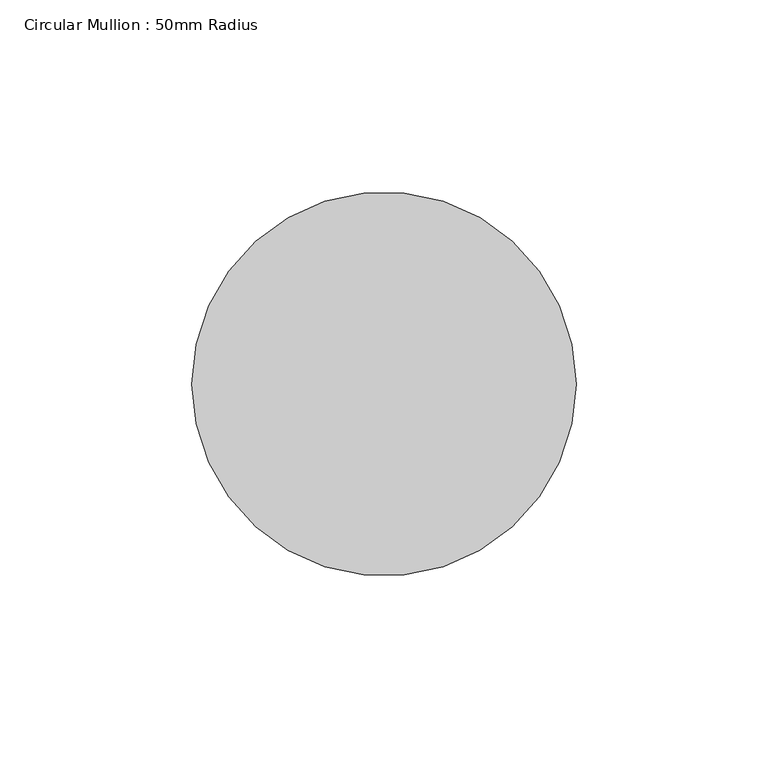
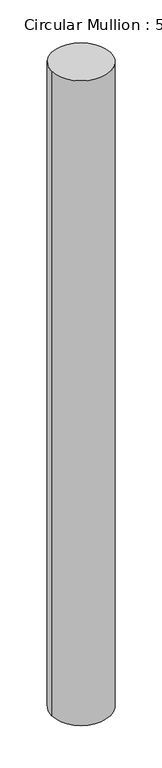
"""IFC4 building model written with IfcOpenShell, lengths in millimetres: member geometry, Circular Mullion : 50mm Radius."""

from ifc_helpers import new_model, si_unit, frame, origin, place, context, project, spatial, ellipse_curve, source, transform, mapped, element, save
from ifc_brep_helpers import plane_surface, cylinder_surface, advanced_brep


def circular_mullion_50mm_radius_0a69bc8c(model_context):
    return source(origin(), model_context, "Body", "AdvancedBrep", [
        advanced_brep(
        [(-100.0, 0.0, 0.8319874), (0.0, 0.0, 0.0), (0.0, 0.0, -1158.0703497), (-100.0, 0.0, -1158.8687099)],
        [
            (0, 1, ellipse_curve(frame((-50.0, 0.0, 0.4159937), z_axis=(-0.008318788476697321, -0.013847806669910945, -0.9998695094904698), x_axis=(-0.5148884069821343, -0.8571049902807197, 0.01615437994128195)), 50.0065254, 50.0)),
            (1, 2),
            (2, 3, ellipse_curve(frame((-50.0, 0.0, -1158.4695298), z_axis=(-0.007982642623571047, -0.013288244084562615, 0.9998798427740674), x_axis=(0.5148937281644346, 0.857113848145521, 0.015501613274298874)), 50.0060086, 50.0)),
            (3, 0),
            (1, 0, ellipse_curve(frame((-50.0, 0.0, 0.4159937), z_axis=(-0.008318788476697321, -0.013847806669910945, -0.9998695094904698), x_axis=(-0.5148884069821343, -0.8571049902807197, 0.01615437994128195)), 50.0065254, 50.0)),
            (3, 2, ellipse_curve(frame((-50.0, 0.0, -1158.4695298), z_axis=(-0.007982642623571047, -0.013288244084562615, 0.9998798427740674), x_axis=(0.5148937281644346, 0.857113848145521, 0.015501613274298874)), 50.0060086, 50.0)),
        ],
        [
            cylinder_surface(frame((-50.0, 0.0, 0.0), z_axis=(0.0, 0.0, 1.0), x_axis=(1.0, 0.0, 0.0)), 50.0),
            plane_surface(frame((-261.2796956, 156.958468, 0.0), z_axis=(0.008318788476697321, 0.013847806669910945, 0.9998695094904698), x_axis=(0.5148884069821359, 0.8571049902807188, -0.016154379941281008))),
            plane_surface(frame((-261.2796956, 156.958468, -1158.0703497), z_axis=(0.007982642623571047, 0.013288244084562615, -0.9998798427740674), x_axis=(0.5148937281644345, 0.8571138481455209, 0.01550161327431976))),
        ],
        [
            (0, [[1, 2, 3, 4]]),
            (0, [[5, -4, 6, -2]]),
            (1, [[-1, -5]]),
            (2, [[-6, -3]]),
        ],
    ),
    ])


if __name__ == "__main__":
    model = new_model("IFC4")
    model_context = context("Model", 3, world=origin())
    ifc_project = project(units=[si_unit("LENGTHUNIT", "METRE", prefix="MILLI")], contexts=[model_context])
    site = spatial("IfcSite", under=ifc_project)
    building = spatial("IfcBuilding", under=site)
    placement = place(None, origin())
    circular_mullion_50mm_radius_shape = circular_mullion_50mm_radius_0a69bc8c(model_context)
    element("IfcMember", 1, ObjectType="Circular Mullion : 50mm Radius", at=placement, inside=building, context=model_context, shape_type="MappedRepresentation", body=[
        mapped(circular_mullion_50mm_radius_shape, transform((0.0, 0.0, 0.0), x_axis=(1.0, 0.0, 0.0), y_axis=(0.0, 1.0, 0.0), z_axis=(0.0, 0.0, 1.0))),
    ])
    save(model, "model.ifc")

# Revit data of these elements
# Type "Circular Mullion : 50mm Radius"
#   built-in parameter 1007350 = 0.164042 (stored number, unit not read)
# Element 1 (IfcMember, "Circular Mullion : 50mm Radius")
#   Materials on its faces: "Aluminium"
# Materials
#   "Aluminium": class "Metal", colour RGB 247 247 247, transparency 0, Description = "Aluminium 6061", Cost = 0
